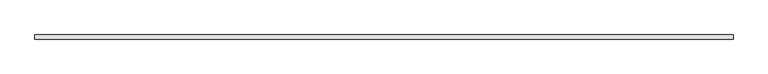
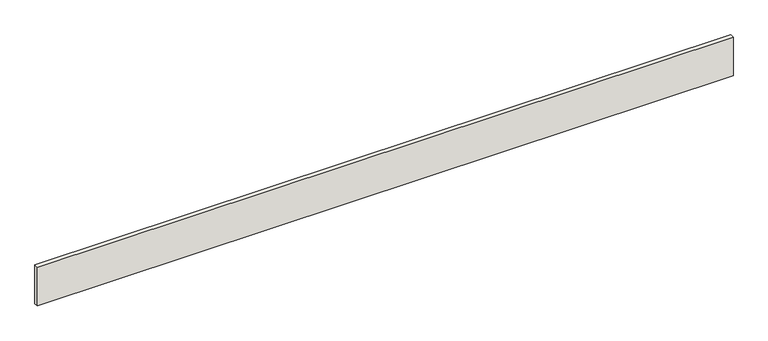
"""IFC4 building model written with IfcOpenShell, lengths in millimetres: wall geometry, Holzwand."""

from ifc_helpers import new_model, si_unit, origin, origin_with_axes, place, context, project, spatial, polyline, outline, extrude, source, transform, mapped, element, save


def wall_0601cf4d(model_context):
    return source(origin(), model_context, "Body", "SweptSolid", [
        extrude(outline(polyline([(0.0, 100.0), (17000.0, 100.0), (17000.0, 0.0), (0.0, 0.0), (0.0, 100.0)])), origin_with_axes(), (0.0, 0.0, 1.0), 1000.0),
    ])


if __name__ == "__main__":
    model = new_model("IFC4")
    model_context = context("Model", 3, world=origin())
    ifc_project = project(units=[si_unit("LENGTHUNIT", "METRE", prefix="MILLI")], contexts=[model_context])
    site = spatial("IfcSite", under=ifc_project)
    building = spatial("IfcBuilding", under=site)
    placement = place(None, origin())
    wall_shape = wall_0601cf4d(model_context)
    element("IfcWall", 1, ObjectType="Holzwand", at=placement, inside=building, context=model_context, shape_type="MappedRepresentation", body=[
        mapped(wall_shape, transform((0.0, 0.0, 0.0), x_axis=(1.0, 0.0, 0.0), y_axis=(0.0, 1.0, 0.0), z_axis=(0.0, 0.0, 1.0))),
    ])
    save(model, "model.ifc")

# Revit data of these elements
# Element 1 (IfcWall, "Holzwand")
#   Materials on its faces: "glas"
# Materials
#   "glas": class "Unassigned", colour RGB 250 253 254, transparency 0.95
